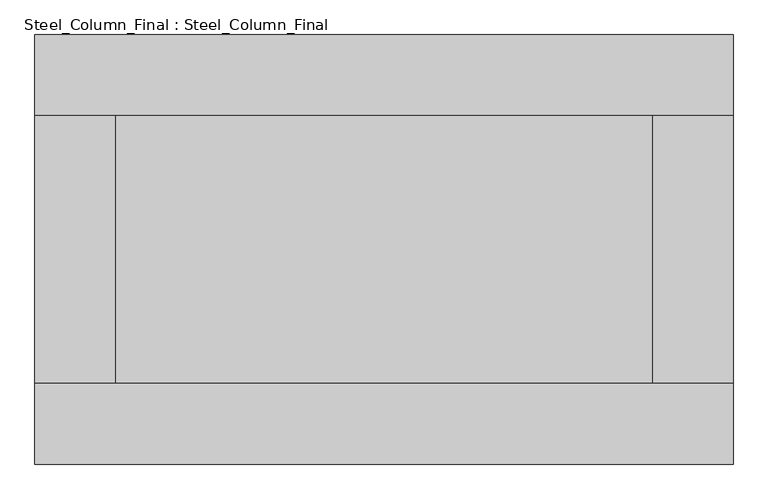
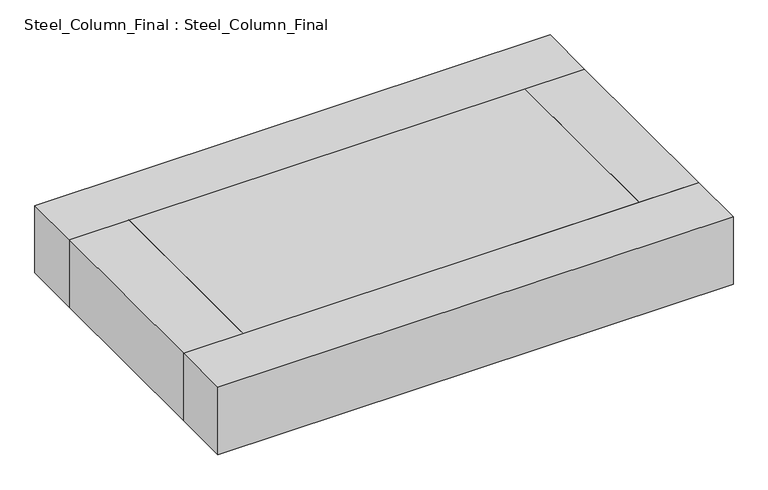
"""IFC4 building model written with IfcOpenShell, lengths in millimetres: proxy geometry, Steel_Column_Final : Steel_Column_Final."""

from ifc_helpers import new_model, si_unit, frame, origin, place, context, project, spatial, polyline, outline, extrude, source, transform, mapped, element, save


def steel_column_final_steel_column_final_c9f65fbe(model_context):
    return source(origin(), model_context, "Body", "SweptSolid", [
        extrude(outline(polyline([(6500.0, 2500.0), (-6500.0, 2500.0), (-6500.0, 4000.0), (6500.0, 4000.0), (6500.0, 2500.0)])), frame((0.0, 0.0, 21310.0), z_axis=(0.0, 0.0, 1.0), x_axis=(1.0, 0.0, 0.0)), (0.0, 0.0, 1.0), 1800.0),
        extrude(outline(polyline([(-6500.0, -2500.0), (6500.0, -2500.0), (6500.0, -4000.0), (-6500.0, -4000.0), (-6500.0, -2500.0)])), frame((0.0, 0.0, 21310.0), z_axis=(0.0, 0.0, 1.0), x_axis=(1.0, 0.0, 0.0)), (0.0, 0.0, 1.0), 1800.0),
        extrude(outline(polyline([(5000.0, -2500.0), (5000.0, 2500.0), (6500.0, 2500.0), (6500.0, -2500.0), (5000.0, -2500.0)])), frame((0.0, 0.0, 21310.0), z_axis=(0.0, 0.0, 1.0), x_axis=(1.0, 0.0, 0.0)), (0.0, 0.0, 1.0), 1800.0),
        extrude(outline(polyline([(-5000.0, 2500.0), (-5000.0, -2500.0), (-6500.0, -2500.0), (-6500.0, 2500.0), (-5000.0, 2500.0)])), frame((0.0, 0.0, 21310.0), z_axis=(0.0, 0.0, 1.0), x_axis=(1.0, 0.0, 0.0)), (0.0, 0.0, 1.0), 1800.0),
        extrude(outline(polyline([(-5000.0, -2500.0), (-5000.0, 2500.0), (5000.0, 2500.0), (5000.0, -2500.0), (-5000.0, -2500.0)])), frame((0.0, 0.0, 21310.0), z_axis=(0.0, 0.0, 1.0), x_axis=(1.0, 0.0, 0.0)), (0.0, 0.0, 1.0), 1800.0),
    ])


if __name__ == "__main__":
    model = new_model("IFC4")
    model_context = context("Model", 3, world=origin())
    ifc_project = project(units=[si_unit("LENGTHUNIT", "METRE", prefix="MILLI")], contexts=[model_context])
    site = spatial("IfcSite", under=ifc_project)
    building = spatial("IfcBuilding", under=site)
    placement = place(None, origin())
    steel_column_final_steel_column_final_shape = steel_column_final_steel_column_final_c9f65fbe(model_context)
    element("IfcBuildingElementProxy", 1, Name="Steel_Column_Final : Steel_Column_Final", ObjectType="Steel_Column_Final : Steel_Column_Final", at=placement, inside=building, context=model_context, shape_type="MappedRepresentation", body=[
        mapped(steel_column_final_steel_column_final_shape, transform((0.0, 0.0, 0.0), x_axis=(1.0, 0.0, 0.0), y_axis=(0.0, 1.0, 0.0), z_axis=(0.0, 0.0, 1.0))),
    ])
    save(model, "model.ifc")

# Revit data of these elements
# Type "Steel_Column_Final : Steel_Column_Final"
#   Top Width [instance default] = 5000 mm
#   Top Length = 10000 mm
#   Length = 21000 mm
#   Height [instance default] = 50000 mm
#   Bottom Width [instance default] = 5000 mm
#   Default Elevation = 0
# Element 1 (IfcBuildingElementProxy, "Steel_Column_Final : Steel_Column_Final")
#   Height = 21310 mm
